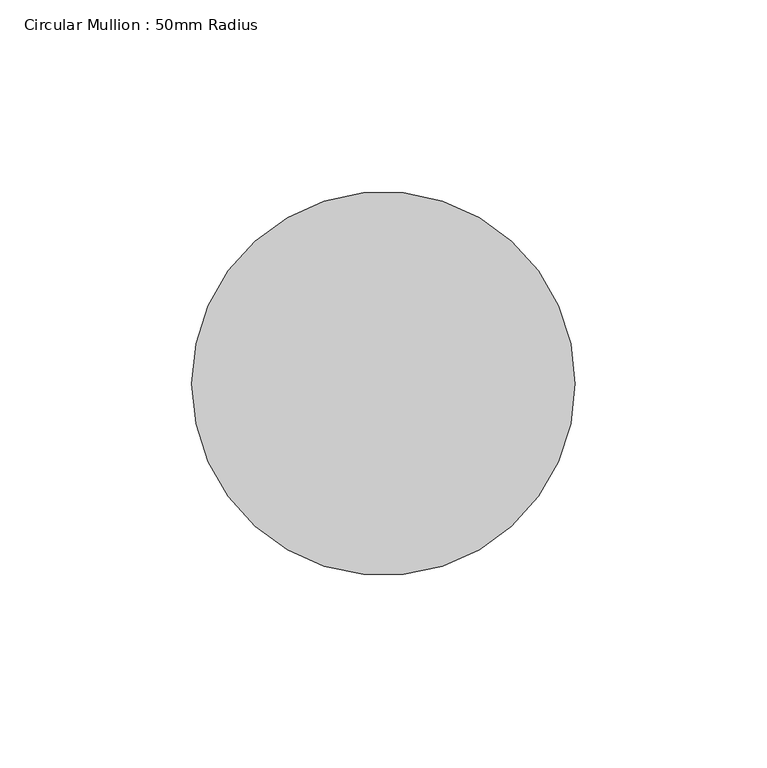
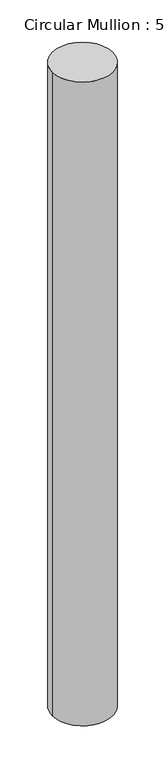
"""IFC4 building model written with IfcOpenShell, lengths in millimetres: member geometry, Circular Mullion : 50mm Radius."""

from ifc_helpers import new_model, si_unit, point, frame, origin, origin_2d, place, context, project, spatial, circle_curve, trimmed, segment, composite_curve, outline, extrude, source, transform, mapped, element, save


def circular_mullion_50mm_radius_a3baa6dd(model_context):
    return source(origin(), model_context, "Body", "SweptSolid", [
        extrude(outline(composite_curve([segment(trimmed(circle_curve(origin_2d(), 50.0), [point((50.0, 0.0))], [point((-50.0, 0.0))], False, "CARTESIAN"), True, "CONTINUOUS"), segment(trimmed(circle_curve(origin_2d(), 50.0), [point((-50.0, 0.0))], [point((50.0, 0.0))], False, "CARTESIAN"), True, "CONTINUOUS")], self_intersect=False)), frame((0.0, 0.0, -1128.1013531), z_axis=(0.0, 0.0, 1.0), x_axis=(1.0, 0.0, 0.0)), (0.0, 0.0, 1.0), 1128.1013531),
    ])


if __name__ == "__main__":
    model = new_model("IFC4")
    model_context = context("Model", 3, world=origin())
    ifc_project = project(units=[si_unit("LENGTHUNIT", "METRE", prefix="MILLI")], contexts=[model_context])
    site = spatial("IfcSite", under=ifc_project)
    building = spatial("IfcBuilding", under=site)
    placement = place(None, origin())
    circular_mullion_50mm_radius_shape = circular_mullion_50mm_radius_a3baa6dd(model_context)
    element("IfcMember", 1, ObjectType="Circular Mullion : 50mm Radius", at=placement, inside=building, context=model_context, shape_type="MappedRepresentation", body=[
        mapped(circular_mullion_50mm_radius_shape, transform((0.0, 0.0, 0.0), x_axis=(1.0, 0.0, 0.0), y_axis=(0.0, 1.0, 0.0), z_axis=(0.0, 0.0, 1.0))),
    ])
    save(model, "model.ifc")

# Revit data of these elements
# Type "Circular Mullion : 50mm Radius"
#   built-in parameter 1007350 = 0.164042 (stored number, unit not read)
# Element 1 (IfcMember, "Circular Mullion : 50mm Radius")
#   Materials on its faces: "Aluminium"
# Materials
#   "Aluminium": class "Metal", colour RGB 247 247 247, transparency 0, Description = "Aluminium 6061", Cost = 0
